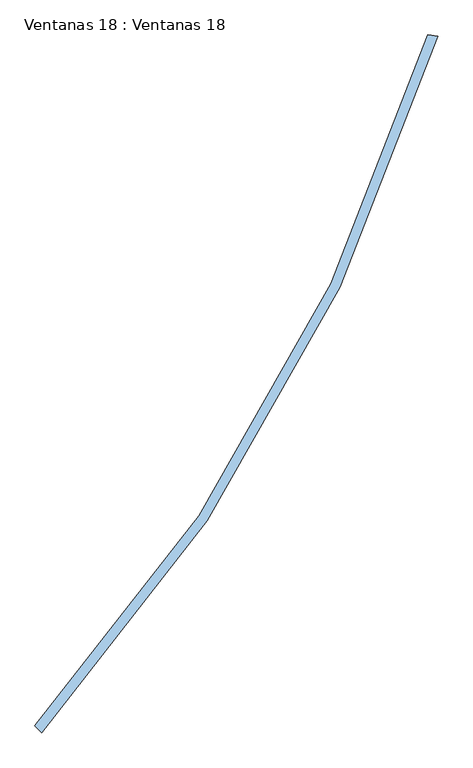
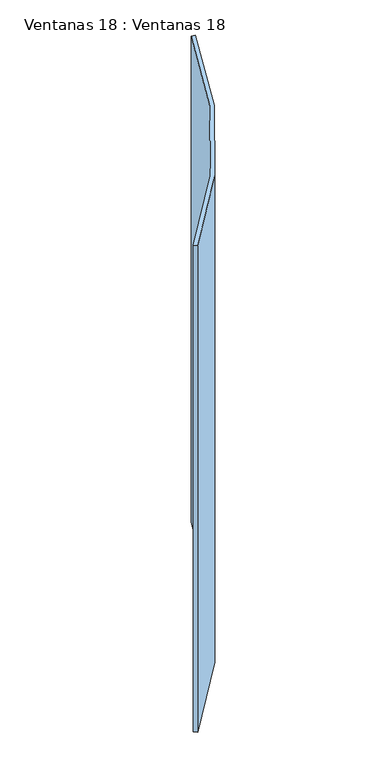
"""IFC4 building model written with IfcOpenShell, lengths in millimetres: window geometry, Ventanas 18 : Ventanas 18."""

from ifc_helpers import new_model, si_unit, point, frame, frame_2d, origin, place, context, project, spatial, polyline, circle_curve, trimmed, segment, composite_curve, outline, extrude, source, transform, mapped, element, save


def ventanas_18_ventanas_18_c769e58a(model_context):
    return source(origin(), model_context, "Body", "SweptSolid", [
        extrude(outline(composite_curve([segment(trimmed(circle_curve(frame_2d((2573.6790405, 3166.0826909)), 3727.0669896), [point((5336.3434329, 664.340538))], [point((6134.9585103, 2066.8480103))], True, "CARTESIAN"), True, "CONTINUOUS"), segment(polyline([(6134.9585103, 2066.8480103), (6154.7122771, 2063.719321)]), True, "CONTINUOUS"), segment(trimmed(circle_curve(frame_2d((2575.1950635, 3164.7517381)), 3745.0254826), [point((6154.7122771, 2063.719321))], [point((5350.4855686, 650.1984024))], False, "CARTESIAN"), True, "CONTINUOUS"), segment(polyline([(5350.4855686, 650.1984024), (5336.3434329, 664.340538)]), True, "CONTINUOUS")], self_intersect=False)), frame((0.0, 0.0, 5100.0), z_axis=(0.0, 0.0, 1.0), x_axis=(1.0, 0.0, 0.0)), (0.0, 0.0, 1.0), 2627.8129716),
    ])


if __name__ == "__main__":
    model = new_model("IFC4")
    model_context = context("Model", 3, world=origin())
    ifc_project = project(units=[si_unit("LENGTHUNIT", "METRE", prefix="MILLI")], contexts=[model_context])
    site = spatial("IfcSite", under=ifc_project)
    building = spatial("IfcBuilding", under=site)
    placement = place(None, origin())
    ventanas_18_ventanas_18_shape = ventanas_18_ventanas_18_c769e58a(model_context)
    element("IfcWindow", 1, ObjectType="Ventanas 18 : Ventanas 18", at=placement, inside=building, context=model_context, shape_type="MappedRepresentation", body=[
        mapped(ventanas_18_ventanas_18_shape, transform((0.0, 0.0, 0.0), x_axis=(1.0, 0.0, 0.0), y_axis=(0.0, 1.0, 0.0), z_axis=(0.0, 0.0, 1.0))),
    ])
    save(model, "model.ifc")

# Revit data of these elements
# Type "Ventanas 18 : Ventanas 18"
#   Type Mark = "44"
# Element 1 (IfcWindow, "Ventanas 18 : Ventanas 18")
#   Materials on its faces: "VIDRIO"
# Materials
#   "VIDRIO": class "Genérico", colour RGB 120 120 120, transparency 0, Cost = 0
